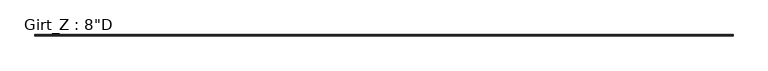
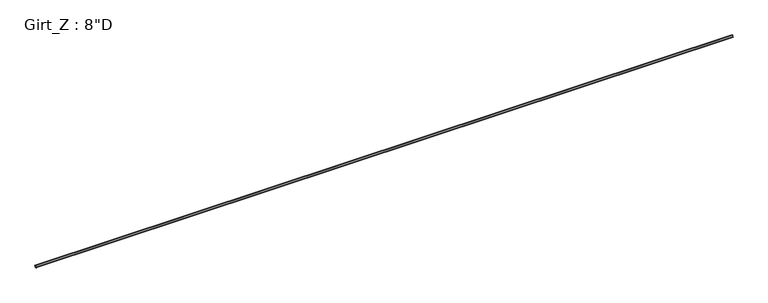
"""IFC4 building model written with IfcOpenShell, lengths in millimetres: beam geometry."""

from ifc_helpers import new_model, si_unit, point, frame, frame_2d, origin, place, context, project, spatial, polyline, circle_curve, trimmed, segment, composite_curve, outline, extrude, source, transform, mapped, element, save


def beam_fce8c877(model_context):
    return source(origin(), model_context, "Body", "SweptSolid", [
        extrude(outline(composite_curve([segment(polyline([(63.5, 101.6), (75.745104, 87.0068534), (73.6169367, 85.221109), (62.204539, 98.821875), (3.3005807, 98.821875)]), True, "CONTINUOUS"), segment(trimmed(circle_curve(frame_2d((3.3741066, 96.8381931)), 1.9850441), [point((3.3005807, 98.821875))], [point((1.3890625, 96.8381931))], True, "CARTESIAN"), True, "CONTINUOUS"), segment(polyline([(1.3890625, 96.8381931), (1.3890625, -96.8375)]), True, "CONTINUOUS"), segment(trimmed(circle_curve(frame_2d((-3.3734375, -96.8375)), 4.7625), [point((1.3890625, -96.8375))], [point((-3.3734375, -101.6))], False, "CARTESIAN"), True, "CONTINUOUS"), segment(polyline([(-3.3734375, -101.6), (-63.5, -101.6), (-75.745104, -87.0068534), (-73.6169367, -85.221109), (-62.204539, -98.821875), (-3.2694106, -98.821875)]), True, "CONTINUOUS"), segment(trimmed(circle_curve(frame_2d((-3.3748024, -96.8389339)), 1.9857399), [point((-3.2694106, -98.821875))], [point((-1.3890625, -96.8389339))], True, "CARTESIAN"), True, "CONTINUOUS"), segment(polyline([(-1.3890625, -96.8389339), (-1.3890625, 96.8375)]), True, "CONTINUOUS"), segment(trimmed(circle_curve(frame_2d((3.3734375, 96.8375)), 4.7625), [point((-1.3890625, 96.8375))], [point((3.3734375, 101.6))], False, "CARTESIAN"), True, "CONTINUOUS"), segment(polyline([(3.3734375, 101.6), (63.5, 101.6)]), True, "CONTINUOUS")], self_intersect=False)), frame((-40666.0697266, 0.0, 0.0), z_axis=(1.0, 0.0, 0.0), x_axis=(0.0, 1.0, 0.0)), (0.0, 0.0, 1.0), 81171.8019531),
    ])


if __name__ == "__main__":
    model = new_model("IFC4")
    model_context = context("Model", 3, world=origin())
    ifc_project = project(units=[si_unit("LENGTHUNIT", "METRE", prefix="MILLI")], contexts=[model_context])
    site = spatial("IfcSite", under=ifc_project)
    building = spatial("IfcBuilding", under=site)
    placement = place(None, origin())
    beam_shape = beam_fce8c877(model_context)
    element("IfcBeam", 1, ObjectType="Girt_Z : 8\"D", at=placement, inside=building, context=model_context, shape_type="MappedRepresentation", body=[
        mapped(beam_shape, transform((0.0, 0.0, 0.0), x_axis=(1.0, 0.0, 0.0), y_axis=(0.0, 1.0, 0.0), z_axis=(0.0, 0.0, 1.0))),
    ])
    save(model, "model.ifc")

# Revit data of these elements
# Type "Girt_Z : 8\"D"
#   Web_Thickness = 0' - 0 7/64"
#   Length [instance default] = 10' - 0"
#   Leg_1 = 0' - 2 1/2"
#   Height = 0' - 8"
#   Structural Material [instance default] = none
# Element 1 (IfcBeam, "Girt_Z : 8\"D")
#   Structural Material = Steel
#   Materials on its faces: "Steel"
# Materials
#   "Steel": class "Metal", colour RGB 118 118 114, transparency 0, Description = "Steel, mill finish", Cost = 0
